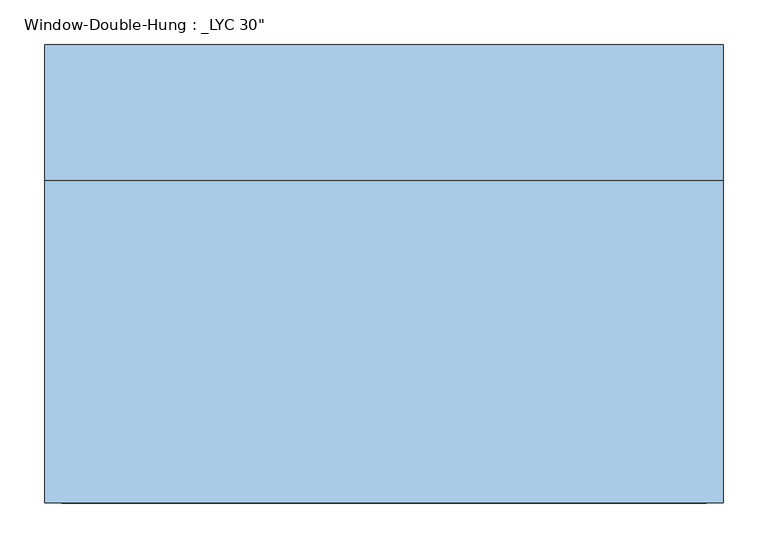
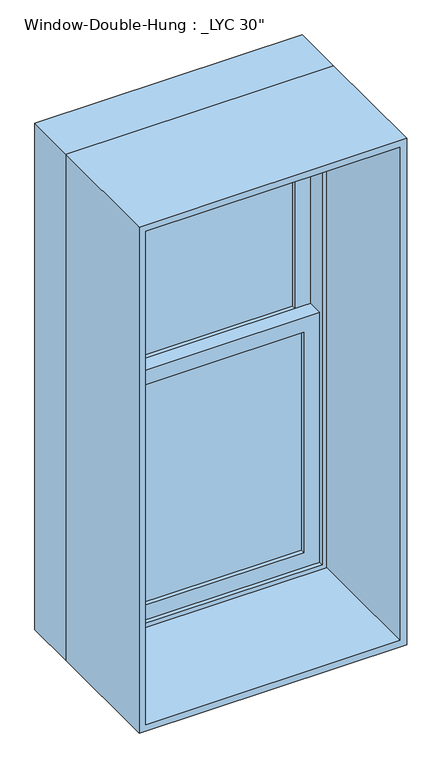
"""IFC4 building model written with IfcOpenShell, lengths in millimetres: window geometry."""

from ifc_helpers import new_model, si_unit, frame, origin, place, context, project, spatial, polyline, outline, extrude, source, transform, mapped, element, save


def window_1a25927d(model_context):
    return source(origin(), model_context, "Body", "SweptSolid", [
        extrude(outline(polyline([(304.8, 158.75), (304.8, 152.4), (-304.8, 152.4), (-304.8, 158.75), (304.8, 158.75)])), frame((0.0, 0.0, 990.6), z_axis=(0.0, 0.0, 1.0), x_axis=(1.0, 0.0, 0.0)), (0.0, 0.0, 1.0), 663.575),
        extrude(outline(polyline([(-304.8, 146.05), (304.8, 146.05), (304.8, 139.7), (-304.8, 139.7), (-304.8, 146.05)])), frame((0.0, 0.0, 990.6), z_axis=(0.0, 0.0, 1.0), x_axis=(1.0, 0.0, 0.0)), (0.0, 0.0, 1.0), 663.575),
        extrude(outline(polyline([(304.8, 203.2), (304.8, 196.85), (-304.8, 196.85), (-304.8, 203.2), (304.8, 203.2)])), frame((0.0, 0.0, 1698.625), z_axis=(0.0, 0.0, 1.0), x_axis=(1.0, 0.0, 0.0)), (0.0, 0.0, 1.0), 663.575),
        extrude(outline(polyline([(-304.8, 190.5), (304.8, 190.5), (304.8, 184.15), (-304.8, 184.15), (-304.8, 190.5)])), frame((0.0, 0.0, 1698.625), z_axis=(0.0, 0.0, 1.0), x_axis=(1.0, 0.0, 0.0)), (0.0, 0.0, 1.0), 663.575),
        extrude(outline(polyline([(1698.625, -349.25), (946.15, -349.25), (946.15, 349.25), (1698.625, 349.25), (1698.625, -349.25)]), holes=[polyline([(1654.175, 304.8), (990.6, 304.8), (990.6, -304.8), (1654.175, -304.8), (1654.175, 304.8)])]), frame((0.0, 127.0, 0.0), z_axis=(0.0, 1.0, 0.0), x_axis=(0.0, 0.0, 1.0)), (0.0, 0.0, 1.0), 44.45),
        extrude(outline(polyline([(2406.65, -349.25), (1654.175, -349.25), (1654.175, 349.25), (2406.65, 349.25), (2406.65, -349.25)]), holes=[polyline([(2362.2, 304.8), (1698.625, 304.8), (1698.625, -304.8), (2362.2, -304.8), (2362.2, 304.8)])]), frame((0.0, 171.45, 0.0), z_axis=(0.0, 1.0, 0.0), x_axis=(0.0, 0.0, 1.0)), (0.0, 0.0, 1.0), 44.45),
        extrude(outline(polyline([(2438.4, -381.0), (914.4, -381.0), (914.4, 381.0), (2438.4, 381.0), (2438.4, -381.0)]), holes=[polyline([(2406.65, 349.25), (946.15, 349.25), (946.15, -349.25), (2406.65, -349.25), (2406.65, 349.25)])]), frame((0.0, 114.3, 0.0), z_axis=(0.0, 1.0, 0.0), x_axis=(0.0, 0.0, 1.0)), (0.0, 0.0, 1.0), 152.4),
        extrude(outline(polyline([(2438.4, 381.0), (2438.4, -381.0), (914.4, -381.0), (914.4, 381.0), (2438.4, 381.0)]), holes=[polyline([(2419.35, 361.95), (933.45, 361.95), (933.45, -361.95), (2419.35, -361.95), (2419.35, 361.95)])]), frame((0.0, -247.65, 0.0), z_axis=(0.0, 1.0, 0.0), x_axis=(0.0, 0.0, 1.0)), (0.0, 0.0, 1.0), 361.95),
    ])


if __name__ == "__main__":
    model = new_model("IFC4")
    model_context = context("Model", 3, world=origin())
    ifc_project = project(units=[si_unit("LENGTHUNIT", "METRE", prefix="MILLI")], contexts=[model_context])
    site = spatial("IfcSite", under=ifc_project)
    building = spatial("IfcBuilding", under=site)
    placement = place(None, origin())
    window_shape = window_1a25927d(model_context)
    element("IfcWindow", 1, ObjectType="Window-Double-Hung : _LYC 30\"", at=placement, inside=building, context=model_context, shape_type="MappedRepresentation", body=[
        mapped(window_shape, transform((0.0, 0.0, 0.0), x_axis=(1.0, 0.0, 0.0), y_axis=(0.0, 1.0, 0.0), z_axis=(0.0, 0.0, 1.0))),
    ])
    save(model, "model.ifc")

# Revit data of these elements
# Type "Window-Double-Hung : _LYC 30\""
#   Type Mark = "19"
#   Fire Rating = "0.5h"
#   Assembly Code = "B2020100"
#   Wall Thickness [instance default] = 0' - 6"
#   Visual Light Transmittance = 0.9
#   Thermal Resistance (R) = 1.8146 (h·ft²·°F)/BTU
#   Solar Heat Gain Coefficient = 0.78
#   Rough Width = 2' - 6 1/2"
#   Rough Height = 5' - 0 1/2"
#   Muntin Width = 2' - 0"
#   Muntin Height = 2' - 2 1/8"
#   Interior Wall Closure [instance default] = 0' - 1 1/2"
#   Heat Transfer Coefficient (U) = 0.6496 BTU/(h·ft²·°F)
#   Frame Extension [instance default] = 0' - 2"
#   Exterior Wall Closure [instance default] = 0' - 0 1/2"
#   Extension Jamb [instance default] = 0' - 0 3/4"
#   Height = 5' - 0"
#   Width = 2' - 6"
#   Window Inset [instance default] = 0' - 0 3/4"
#   Top Muntin Visibility = yes
#   Interior Trim Visibility [instance default] = yes
#   Indicator Visibility [instance default] = yes
#   Exterior Trim Visibility [instance default] = yes
#   Extension Jamb Visibility [instance default] = yes
#   Define Thermal Properties by = 1
#   Bottom Muntin Visibility = yes
#   Muntin Pattern = Muntin Pattern_2x2 : Muntin Pattern_2x2
#   Interior Trim Material = Wood - Stained
#   Interior Trim = Trim-Window-Interior-Flat : Picture Frame
#   Interior Frame Material = Wood - Stained
#   Glass Panel Material = Glass
#   Exterior Trim Material = Clad - White
#   Exterior Trim = Trim-Window-Exterior-Flat : with Sill
#   Exterior Frame Material = Clad - White
#   Construction Type Id = ""
#   Wall Closure = (empty or 0)
#   Analytic Construction = (empty or 0)
# Element 1 (IfcWindow, "Window-Double-Hung : _LYC 30\"")
#   Wall Thickness = 1' - 7 1/2"
#   Extension Jamb = 1' - 2 1/4"
#   Materials on its faces: "Wood - Stained", "Glass", "Clad - White"
# Materials
#   "Wood - Stained": class "Wood", colour RGB 224 178 126, transparency 0, Cost = 0
#   "Glass": class "Unassigned", colour RGB 0 128 192, transparency 0.75
#   "Clad - White": class "Wood", colour RGB 242 242 238, transparency 0, Cost = 0
